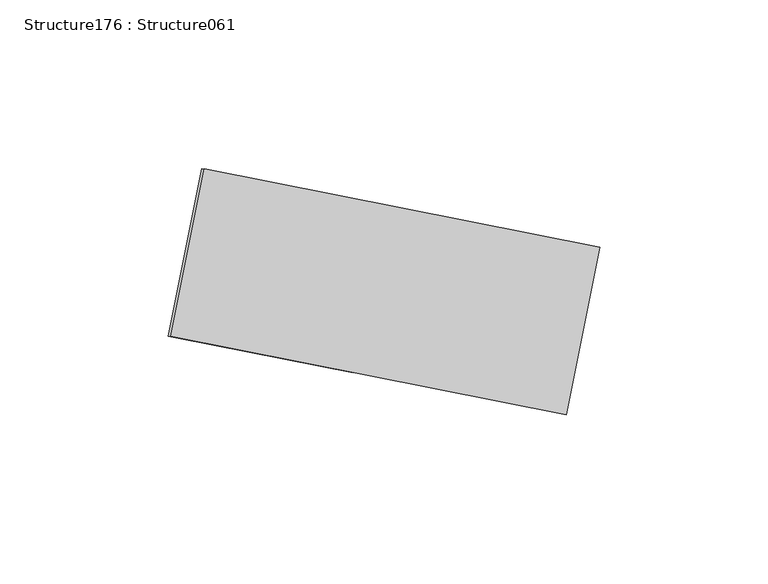
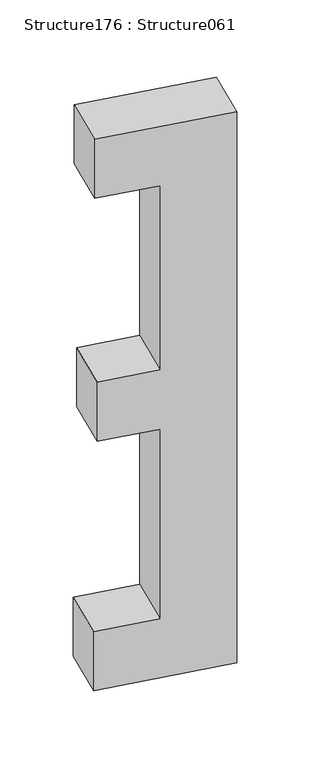
"""IFC4 building model written with IfcOpenShell, lengths in millimetres: proxy geometry, Structure176 : Structure061."""

from ifc_helpers import new_model, si_unit, frame, origin, place, context, project, spatial, polyline, outline, extrude, source, transform, mapped, element, save


def structure176_structure061_e2fd3c83(model_context):
    return source(origin(), model_context, "Body", "SweptSolid", [
        extrude(outline(polyline([(537.7810299, 0.0), (537.7810299, -119.8504949), (480.1634256, -119.8504949), (480.1634256, -64.5410675), (300.3875053, -64.5410675), (300.3875053, -117.5426738), (242.7702568, -117.5426738), (242.7702568, -64.5410675), (57.6168926, -64.5410675), (57.6168926, -120.6165663), (0.0, -120.6165663), (0.0, 0.0), (537.7810299, 0.0)])), frame((-3013.2730604, 235066.4880491, 595.2038833), z_axis=(0.19466222296394123, 0.9808703374813295, 0.0), x_axis=(0.0, 0.0, 1.0)), (0.0, 0.0, 1.0), 50.8),
    ])


if __name__ == "__main__":
    model = new_model("IFC4")
    model_context = context("Model", 3, world=origin())
    ifc_project = project(units=[si_unit("LENGTHUNIT", "METRE", prefix="MILLI")], contexts=[model_context])
    site = spatial("IfcSite", under=ifc_project)
    building = spatial("IfcBuilding", under=site)
    placement = place(None, origin())
    structure176_structure061_shape = structure176_structure061_e2fd3c83(model_context)
    element("IfcBuildingElementProxy", 1, Name="Structure176 : Structure061", ObjectType="Structure176 : Structure061", at=placement, inside=building, context=model_context, shape_type="MappedRepresentation", body=[
        mapped(structure176_structure061_shape, transform((0.0, 0.0, 0.0), x_axis=(1.0, 0.0, 0.0), y_axis=(0.0, 1.0, 0.0), z_axis=(0.0, 0.0, 1.0))),
    ])
    save(model, "model.ifc")

# Revit data of these elements
# Type "Structure176 : Structure061"
#   NameOverride = "Structure061"
# Element 1 (IfcBuildingElementProxy, "Structure176 : Structure061")
#   Materials on its faces: "BRUSHED ALUMINUM LETTERING"
# Materials
#   "BRUSHED ALUMINUM LETTERING": class "Unassigned", colour RGB 169 181 186, transparency 0, Cost = 0
